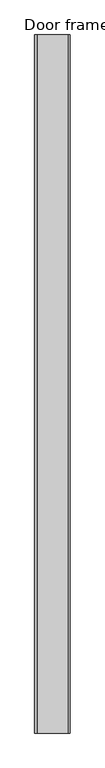
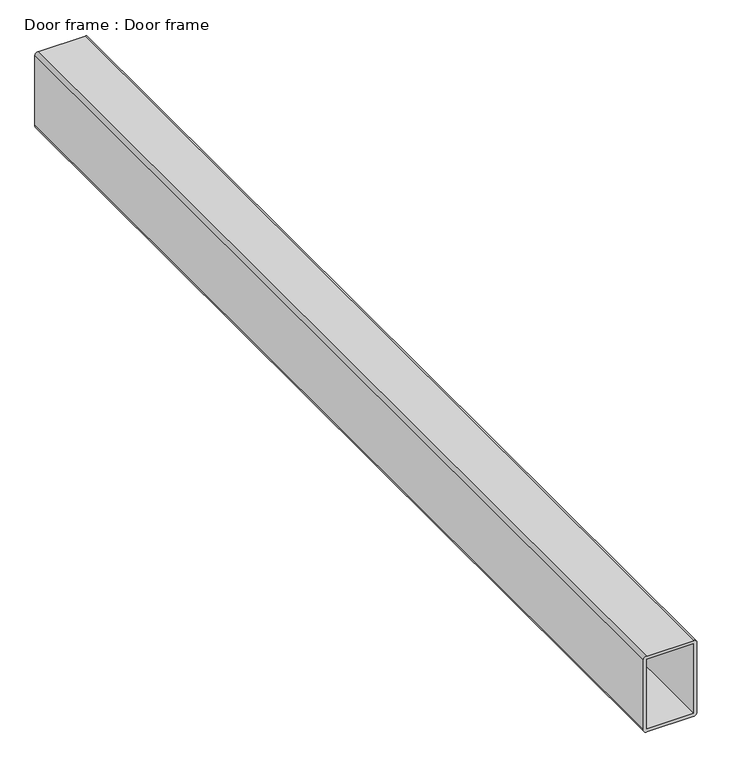
"""IFC4 building model written with IfcOpenShell, lengths in millimetres: proxy geometry, Door frame : Door frame."""

import ifcopenshell
import ifcopenshell.guid

model = None  # the IFC model being written
_history = None  # IfcOwnerHistory: only IFC2X3 demands one
_inside = {}  # id of a spatial element -> (the spatial element, [elements in it])
_under = {}  # id of a project, library or spatial element -> (it, [spatial elements below it])
_declared = {}  # id of a project -> (the project, [libraries it declares])
_typed = {}  # id of a type object -> (the type object, [elements of that type])
_made_of = {}  # id of a material, layer set ... -> (it, [elements and type objects made of it])


def new_model(schema):
    """Start an empty IFC model of exactly this schema.

    Asked for "IFC4X3", IfcOpenShell would pick the latest addendum, in which some entities
    have other attributes; the version numbers below select the first issue.
    IFC2X3 requires an IfcOwnerHistory on every rooted entity: one is made here for all.
    """
    global model, _history
    if schema == "IFC4X3":
        model = ifcopenshell.file(schema_version=(4, 3, 0, 0))
    else:
        model = ifcopenshell.file(schema=schema)
    _inside.clear()
    _under.clear()
    _declared.clear()
    _typed.clear()
    _made_of.clear()
    _history = None
    if model.schema == "IFC2X3":
        org = make("IfcOrganization", Name="unknown")
        user = make(
            "IfcPersonAndOrganization",
            ThePerson=make("IfcPerson", FamilyName="unknown"),
            TheOrganization=org,
        )
        app = make(
            "IfcApplication",
            ApplicationDeveloper=org,
            Version="unknown",
            ApplicationFullName="unknown",
            ApplicationIdentifier="unknown",
        )
        _history = make(
            "IfcOwnerHistory",
            OwningUser=user,
            OwningApplication=app,
            ChangeAction="ADDED",
            CreationDate=0,
        )
    return model


def make(cls, **values):
    """One entity of the class cls with the attributes given. An attribute that is None is left unset."""
    return model.create_entity(
        cls, **{name: value for name, value in values.items() if value is not None}
    )


def rooted(cls, **values):
    """An entity with a GlobalId (a new one), such as an element, a storey or a relation."""
    return make(cls, GlobalId=ifcopenshell.guid.new(), OwnerHistory=_history, **values)


def si_unit(unit_type, name, prefix=None):
    """IfcSIUnit, for example si_unit("LENGTHUNIT", "METRE", prefix="MILLI")."""
    return make("IfcSIUnit", UnitType=unit_type, Prefix=prefix, Name=name)


def assignment(units):
    """IfcUnitAssignment: the units of a project."""
    return None if units is None else make("IfcUnitAssignment", Units=units)


def point(xyz):
    """IfcCartesianPoint."""
    return None if xyz is None else make("IfcCartesianPoint", Coordinates=xyz)


def direction(xyz):
    """IfcDirection."""
    return None if xyz is None else make("IfcDirection", DirectionRatios=xyz)


def frame(location, z_axis=None, x_axis=None):
    """IfcAxis2Placement3D, a coordinate frame: its origin and axes. An axis left out is left unset."""
    return make(
        "IfcAxis2Placement3D",
        Location=point(location),
        Axis=direction(z_axis),
        RefDirection=direction(x_axis),
    )


def frame_2d(location, x_axis=None):
    """IfcAxis2Placement2D, a coordinate frame in the plane: its origin and x axis."""
    return make(
        "IfcAxis2Placement2D", Location=point(location), RefDirection=direction(x_axis)
    )


def origin():
    """The frame at (0, 0, 0) with its axes left unset."""
    return frame((0.0, 0.0, 0.0))


def place(relative_to, where):
    """IfcLocalPlacement: puts the frame where relative to a parent placement (None: the world)."""
    return make(
        "IfcLocalPlacement", PlacementRelTo=relative_to, RelativePlacement=where
    )


def context(
    kind, dimensions, precision=None, world=None, true_north=None, identifier=None
):
    """IfcGeometricRepresentationContext, for example the 3D "Model" context."""
    return make(
        "IfcGeometricRepresentationContext",
        ContextIdentifier=identifier,
        ContextType=kind,
        CoordinateSpaceDimension=dimensions,
        Precision=precision,
        WorldCoordinateSystem=world,
        TrueNorth=true_north,
    )


def project(units=None, contexts=None):
    """IfcProject with its units and contexts."""
    return rooted(
        "IfcProject",
        Name="project",
        RepresentationContexts=contexts,
        UnitsInContext=assignment(units),
    )


def spatial(cls, under=None, at=None, **own):
    """A site, building, storey or space (cls), placed at a placement, below another one or the project."""
    s = rooted(cls, ObjectPlacement=at, **own)
    if under is not None:
        _under.setdefault(under.id(), (under, []))[1].append(s)
    return s


def polyline(points):
    """IfcPolyline through the points."""
    return make("IfcPolyline", Points=[point(p) for p in points])


def circle_curve(where, radius):
    """IfcCircle in the frame where."""
    return make("IfcCircle", Position=where, Radius=radius)


def trimmed(basis, trim1, trim2, sense, master):
    """IfcTrimmedCurve: the piece of a basis curve between two trims."""
    return make(
        "IfcTrimmedCurve",
        BasisCurve=basis,
        Trim1=trim1,
        Trim2=trim2,
        SenseAgreement=sense,
        MasterRepresentation=master,
    )


def segment(curve, same_sense, transition):
    """IfcCompositeCurveSegment."""
    return make(
        "IfcCompositeCurveSegment",
        Transition=transition,
        SameSense=same_sense,
        ParentCurve=curve,
    )


def composite_curve(segments, self_intersect=None):
    """IfcCompositeCurve: segments joined end to end."""
    return make("IfcCompositeCurve", Segments=segments, SelfIntersect=self_intersect)


def outline(outer, holes=None, kind="AREA"):
    """IfcArbitraryClosedProfileDef: a profile drawn as a closed curve; with holes, ...WithVoids."""
    if holes is None:
        return make("IfcArbitraryClosedProfileDef", ProfileType=kind, OuterCurve=outer)
    return make(
        "IfcArbitraryProfileDefWithVoids",
        ProfileType=kind,
        OuterCurve=outer,
        InnerCurves=holes,
    )


def extrude(swept, where, along, depth):
    """IfcExtrudedAreaSolid: the profile swept, set in the frame where, extruded along a direction by depth."""
    return make(
        "IfcExtrudedAreaSolid",
        SweptArea=swept,
        Position=where,
        ExtrudedDirection=direction(along),
        Depth=depth,
    )


def shape(context_of_items, identifier, shape_type, items):
    """IfcShapeRepresentation: the items that make up one representation, for example the "Body"."""
    return make(
        "IfcShapeRepresentation",
        ContextOfItems=context_of_items,
        RepresentationIdentifier=identifier,
        RepresentationType=shape_type,
        Items=items,
    )


def source(mapping_origin, context_of_items, identifier, shape_type, items):
    """IfcRepresentationMap: a shape defined once, which mapped items show again and again."""
    return make(
        "IfcRepresentationMap",
        MappingOrigin=mapping_origin,
        MappedRepresentation=shape(context_of_items, identifier, shape_type, items),
    )


def transform(
    local_origin,
    x_axis=None,
    y_axis=None,
    z_axis=None,
    scale=None,
    scale2=None,
    scale3=None,
    uniform=True,
):
    """IfcCartesianTransformationOperator3D, or its non-uniform kind. x_axis, y_axis, z_axis: its Axis1, 2, 3."""
    if uniform:
        return make(
            "IfcCartesianTransformationOperator3D",
            Axis1=direction(x_axis),
            Axis2=direction(y_axis),
            LocalOrigin=point(local_origin),
            Scale=scale,
            Axis3=direction(z_axis),
        )
    return make(
        "IfcCartesianTransformationOperator3DnonUniform",
        Axis1=direction(x_axis),
        Axis2=direction(y_axis),
        LocalOrigin=point(local_origin),
        Scale=scale,
        Axis3=direction(z_axis),
        Scale2=scale2,
        Scale3=scale3,
    )


def mapped(mapping_source, mapping_target):
    """IfcMappedItem: shows the shape of a source again, moved by a transform."""
    return make(
        "IfcMappedItem", MappingSource=mapping_source, MappingTarget=mapping_target
    )


def made_of(thing, what):
    """Note that an element or type object is made of a material, layer set ...; save() writes the relation."""
    if what is not None:
        _made_of.setdefault(what.id(), (what, []))[1].append(thing)
    return thing


def element(
    cls,
    number,
    at=None,
    inside=None,
    cuts=None,
    type_object=None,
    material=None,
    context=None,
    identifier="Body",
    shape_type=None,
    held_by="IfcProductDefinitionShape",
    body=None,
    shapes=None,
    **own,
):
    """One element of the class cls, such as IfcWall. Its Tag is "e" and its number.

    at: its placement. inside: the storey or other place that contains it. cuts: it is an
    opening in that element (IfcRelVoidsElement). A single representation is given by context,
    identifier, shape_type and body (its items); several are given by shapes. held_by: the class
    of the entity that holds the representations. save() writes the other relations.
    """
    e = rooted(cls, Tag="e%d" % number, ObjectPlacement=at, **own)
    if body is not None:
        shapes = [shape(context, identifier, shape_type, body)]
    if shapes is not None:
        e.Representation = make(held_by, Representations=shapes)
    if inside is not None:
        _inside.setdefault(inside.id(), (inside, []))[1].append(e)
    if cuts is not None:
        rooted(
            "IfcRelVoidsElement", RelatingBuildingElement=cuts, RelatedOpeningElement=e
        )
    if type_object is not None:
        _typed.setdefault(type_object.id(), (type_object, []))[1].append(e)
    return made_of(e, material)


def aggregate(whole, parts):
    """IfcRelAggregates: a whole, such as a stair, and the parts it consists of."""
    return rooted("IfcRelAggregates", RelatingObject=whole, RelatedObjects=parts)


def save(model, path):
    """Write the relations noted so far, then the file.

    IfcRelAggregates (storeys below a building ...), IfcRelContainedInSpatialStructure (elements
    in a storey), IfcRelDefinesByType, IfcRelAssociatesMaterial and IfcRelDeclares: one each for
    every whole, place, type object, material and project.
    """
    for whole, parts in _under.values():
        aggregate(whole, parts)
    for where, things in _inside.values():
        rooted(
            "IfcRelContainedInSpatialStructure",
            RelatedElements=things,
            RelatingStructure=where,
        )
    for kind, things in _typed.values():
        rooted("IfcRelDefinesByType", RelatedObjects=things, RelatingType=kind)
    for what, things in _made_of.values():
        rooted("IfcRelAssociatesMaterial", RelatedObjects=things, RelatingMaterial=what)
    for by, libraries in _declared.values():
        rooted("IfcRelDeclares", RelatingContext=by, RelatedDefinitions=libraries)
    model.write(path)


def door_frame_door_frame_b90efb81(model_context):
    return source(origin(), model_context, "Body", "SweptSolid", [
        extrude(outline(composite_curve([segment(polyline([(34855.8775473, -8390.3106967), (34855.8775473, -8301.4106967)]), True, "CONTINUOUS"), segment(trimmed(circle_curve(frame_2d((34862.2275473, -8301.4106967)), 6.35), [point((34855.8775473, -8301.4106967))], [point((34862.2275473, -8295.0606967))], False, "CARTESIAN"), True, "CONTINUOUS"), segment(polyline([(34862.2275473, -8295.0606967), (35001.9275473, -8295.0606967)]), True, "CONTINUOUS"), segment(trimmed(circle_curve(frame_2d((35001.9275473, -8301.4106967)), 6.35), [point((35001.9275473, -8295.0606967))], [point((35008.2775473, -8301.4106967))], False, "CARTESIAN"), True, "CONTINUOUS"), segment(polyline([(35008.2775473, -8301.4106967), (35008.2775473, -8390.3106967)]), True, "CONTINUOUS"), segment(trimmed(circle_curve(frame_2d((35001.9275473, -8390.3106967)), 6.35), [point((35008.2775473, -8390.3106967))], [point((35001.9275473, -8396.6606967))], False, "CARTESIAN"), True, "CONTINUOUS"), segment(polyline([(35001.9275473, -8396.6606967), (34862.2275473, -8396.6606967)]), True, "CONTINUOUS"), segment(trimmed(circle_curve(frame_2d((34862.2275473, -8390.3106967)), 6.35), [point((34862.2275473, -8396.6606967))], [point((34855.8775473, -8390.3106967))], False, "CARTESIAN"), True, "CONTINUOUS")], self_intersect=False), holes=[polyline([(35001.7775473, -8301.5606967), (34862.3775473, -8301.5606967), (34862.3775473, -8390.1606967), (35001.7775473, -8390.1606967), (35001.7775473, -8301.5606967)])]), frame((0.0, 4540.4513244, 0.0), z_axis=(0.0, 1.0, 0.0), x_axis=(0.0, 0.0, 1.0)), (0.0, 0.0, 1.0), 2000.0),
    ])


if __name__ == "__main__":
    model = new_model("IFC4")
    model_context = context("Model", 3, world=origin())
    ifc_project = project(units=[si_unit("LENGTHUNIT", "METRE", prefix="MILLI")], contexts=[model_context])
    site = spatial("IfcSite", under=ifc_project)
    building = spatial("IfcBuilding", under=site)
    placement = place(None, origin())
    door_frame_door_frame_shape = door_frame_door_frame_b90efb81(model_context)
    element("IfcBuildingElementProxy", 1, Name="Door frame : Door frame", ObjectType="Door frame : Door frame", at=placement, inside=building, context=model_context, shape_type="MappedRepresentation", body=[
        mapped(door_frame_door_frame_shape, transform((0.0, 0.0, 0.0), x_axis=(1.0, 0.0, 0.0), y_axis=(0.0, 1.0, 0.0), z_axis=(0.0, 0.0, 1.0))),
    ])
    save(model, "model.ifc")

# Revit data of these elements
# Type "Door frame : Door frame"
#   NameOverride = "Door frame"
# Element 1 (IfcBuildingElementProxy, "Door frame : Door frame")
#   Materials on its faces: "DOOR FRAME: TUBE STEEL PROFILE - METALIZED, PRIMED & PAINTED (COLOR PER ARCHITECT)"
# Materials
#   "DOOR FRAME: TUBE STEEL PROFILE - METALIZED, PRIMED & PAINTED (COLOR PER ARCHITECT)": class "Unassigned", colour RGB 128 128 128, transparency 0, Cost = 0
